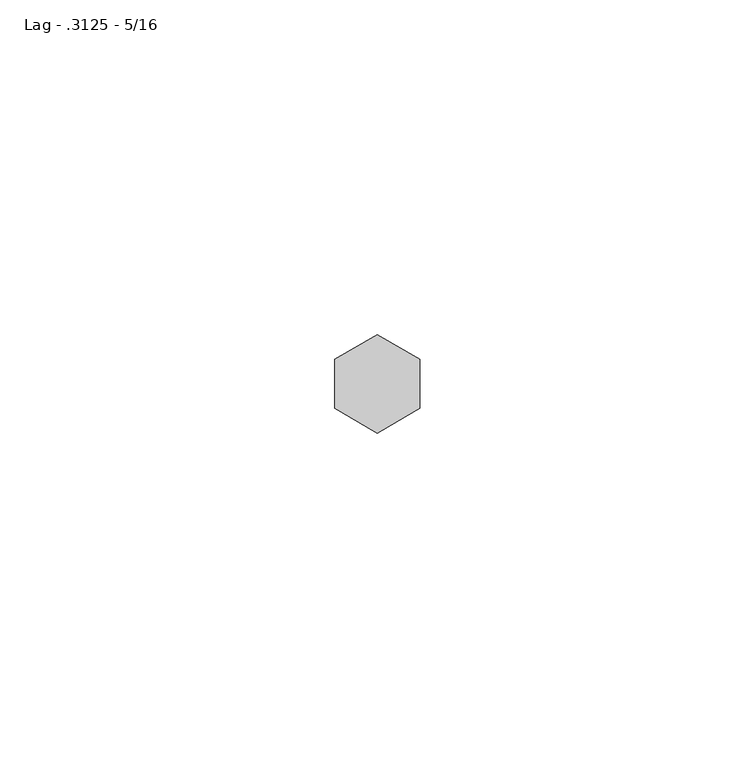
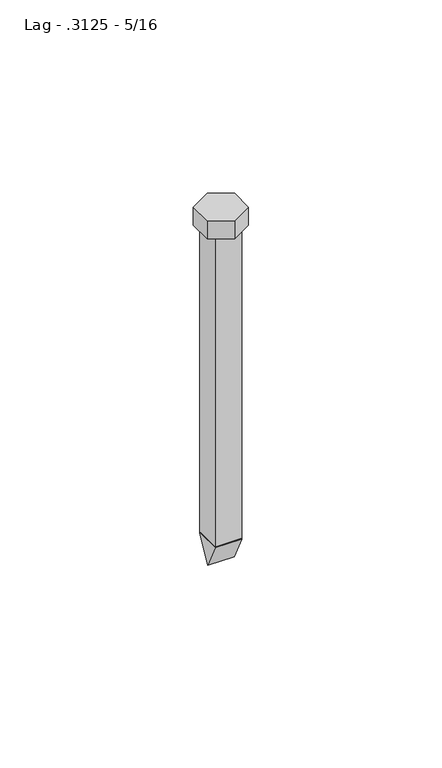
"""IFC4 building model written with IfcOpenShell, lengths in millimetres: fastener geometry, 060523 - W_P_C - Fastenings - Generic - SQUARE : Lag - .3125 - 5/16."""

from ifc_helpers import new_model, si_unit, frame, origin, origin_with_axes, place, context, project, spatial, polyline, outline, extrude, source, transform, mapped, element, save


def lag_3125_5_16_b9fc9e3e(model_context):
    return source(origin(), model_context, "Body", "SweptSolid", [
        extrude(outline(polyline([(0.0, -109.8296), (-4.1148, -101.6), (4.1148, -101.6), (0.0, -109.8296)])), frame((-4.1148, 0.0, 0.0), z_axis=(1.0, 0.0, 0.0), x_axis=(0.0, 1.0, 0.0)), (0.0, 0.0, 1.0), 8.2296),
        extrude(outline(polyline([(-6.35, 3.6661742), (0.0, 7.3323484), (6.35, 3.6661742), (6.35, -3.6661742), (0.0, -7.3323484), (-6.35, -3.6661742), (-6.35, 3.6661742)])), origin_with_axes(), (0.0, 0.0, 1.0), 5.953125),
        extrude(outline(polyline([(-4.1148, 4.1148), (4.1148, 4.1148), (4.1148, -4.1148), (-4.1148, -4.1148), (-4.1148, 4.1148)])), frame((0.0, 0.0, -101.6), z_axis=(0.0, 0.0, 1.0), x_axis=(1.0, 0.0, 0.0)), (0.0, 0.0, 1.0), 101.6),
    ])


if __name__ == "__main__":
    model = new_model("IFC4")
    model_context = context("Model", 3, world=origin())
    ifc_project = project(units=[si_unit("LENGTHUNIT", "METRE", prefix="MILLI")], contexts=[model_context])
    site = spatial("IfcSite", under=ifc_project)
    building = spatial("IfcBuilding", under=site)
    placement = place(None, origin())
    lag_3125_5_16_shape = lag_3125_5_16_b9fc9e3e(model_context)
    element("IfcFastener", 1, ObjectType="060523 - W_P_C - Fastenings - Generic - SQUARE : Lag - .3125 - 5/16", at=placement, inside=building, context=model_context, shape_type="MappedRepresentation", body=[
        mapped(lag_3125_5_16_shape, transform((0.0, 0.0, 0.0), x_axis=(1.0, 0.0, 0.0), y_axis=(0.0, 1.0, 0.0), z_axis=(0.0, 0.0, 1.0))),
    ])
    save(model, "model.ifc")

# Revit data of these elements
# Type "060523 - W_P_C - Fastenings - Generic - SQUARE : Lag - .3125 - 5/16"
#   Washer_Thickness = 0' - 0 5/64"
#   Washer Radius = 0' - 0.39638"
#   Washer Offset - Head = 0' - 0"
#   Washer Offset = 0' - 0"
#   Thickness_of_Substrate [instance default] = 0' - 1"
#   Side = 0' - 0 37/128"
#   Radius = 0' - 0.162"
#   Length [instance default] = 0' - 4"
#   Head Size = 0' - 0 1/2"
#   Head Radius = 0' - 0 1/4"
#   Head Height = 0' - 0 15/64"
#   Double Diameter = 0' - 0.648"
#   Diameter = 0' - 0.324"
#   Default Elevation = 4' - 0"
#   Washer_Nut_Visibility = no
#   Washer_Head_Visibility = no
#   Round_Head_Visibility = no
#   Point Visibility = yes
#   Nut_Visibility = no
#   Hex_Head_Visiblilty = yes
#   Washer Material = none
#   Bolt Material (Size) = AT SILL - FASTENER AT 24" O.C.
# Element 1 (IfcFastener, "060523 - W_P_C - Fastenings - Generic - SQUARE : Lag - .3125 - 5/16")
#   Materials on its faces: "AT SILL - FASTENER AT 24\" O.C."
# Materials
#   "AT SILL - FASTENER AT 24\" O.C.": class "Generic", colour RGB 120 120 120, transparency 0, Cost = 0
